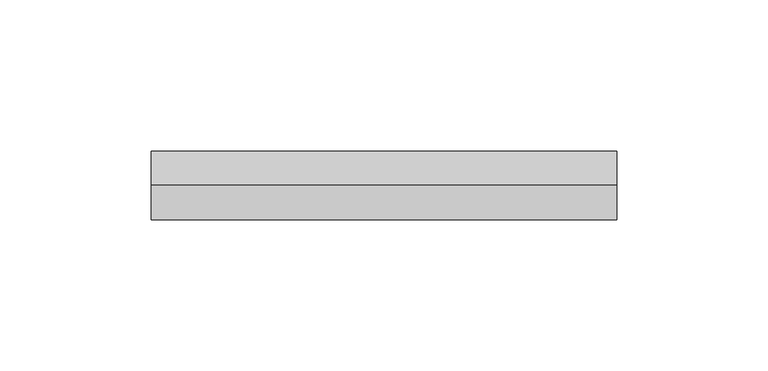
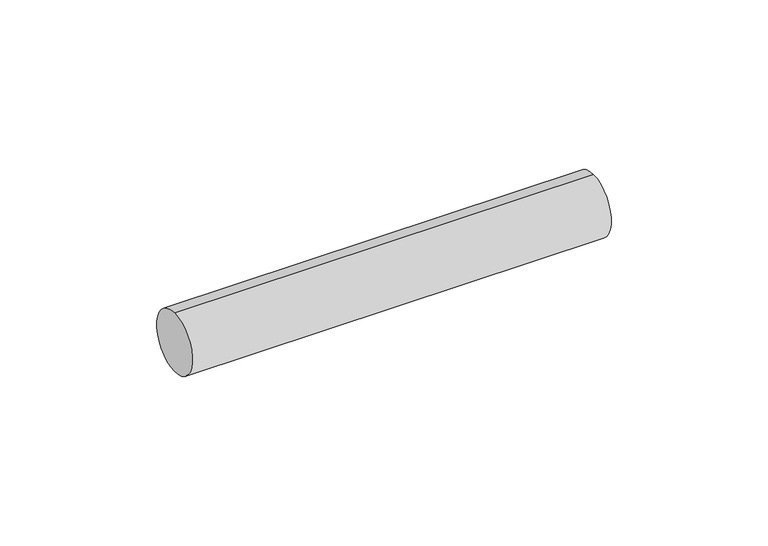
"""IFC4 building model written with IfcOpenShell, lengths in millimetres: proxy geometry, Bolt26:Bolt003:304710 : Bolt26:Bolt003:304710."""

from ifc_helpers import new_model, si_unit, point, frame, frame_2d, origin, place, context, project, spatial, circle_curve, trimmed, segment, composite_curve, outline, extrude, source, transform, mapped, element, save


def generic_models_f7951d7f(model_context):
    return source(origin(), model_context, "Body", "SweptSolid", [
        extrude(outline(composite_curve([segment(trimmed(circle_curve(frame_2d((2174.9207483, 39910.0063132)), 11.4045168), [point((2174.9207483, 39921.41083))], [point((2174.9207483, 39898.6017964))], False, "CARTESIAN"), True, "CONTINUOUS"), segment(trimmed(circle_curve(frame_2d((2174.9207483, 39910.0063132)), 11.4045168), [point((2174.9207483, 39898.6017964))], [point((2174.9207483, 39921.41083))], False, "CARTESIAN"), True, "CONTINUOUS")], self_intersect=False)), frame((15064.3231907, 0.0, 0.0), z_axis=(1.0, 0.0, 0.0), x_axis=(0.0, 1.0, 0.0)), (0.0, 0.0, 1.0), 154.0602393),
    ])


if __name__ == "__main__":
    model = new_model("IFC4")
    model_context = context("Model", 3, world=origin())
    ifc_project = project(units=[si_unit("LENGTHUNIT", "METRE", prefix="MILLI")], contexts=[model_context])
    site = spatial("IfcSite", under=ifc_project)
    building = spatial("IfcBuilding", under=site)
    placement = place(None, origin())
    generic_models_shape = generic_models_f7951d7f(model_context)
    element("IfcBuildingElementProxy", 1, Name="Bolt26:Bolt003:304710 : Bolt26:Bolt003:304710", ObjectType="Bolt26:Bolt003:304710 : Bolt26:Bolt003:304710", at=placement, inside=building, context=model_context, shape_type="MappedRepresentation", body=[
        mapped(generic_models_shape, transform((0.0, 0.0, 0.0), x_axis=(1.0, 0.0, 0.0), y_axis=(0.0, 1.0, 0.0), z_axis=(0.0, 0.0, 1.0))),
    ])
    save(model, "model.ifc")

# Revit data of these elements
# Type "Bolt26:Bolt003:304710 : Bolt26:Bolt003:304710"
#   NameOverride = "Bolt26:Bolt003:304710"
#   ObjectTypeOverride = "Bolt26:Bolt003"
#   Reference = "Bolt003"
#   Category = "Generic Models"
#   Tag = "304710"
# Element 1 (IfcBuildingElementProxy, "Bolt26:Bolt003:304710 : Bolt26:Bolt003:304710")
#   Materials on its faces: "TUBE STEEL STRINGER WELDED TO ANCHORED STEEL PLATE - SEE STRUCT DWGS"
# Materials
#   "TUBE STEEL STRINGER WELDED TO ANCHORED STEEL PLATE - SEE STRUCT DWGS": class "Unassigned", colour RGB 128 128 128, transparency 0, Cost = 0
